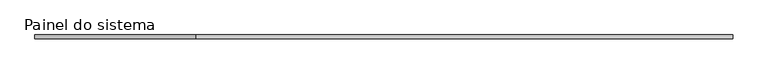
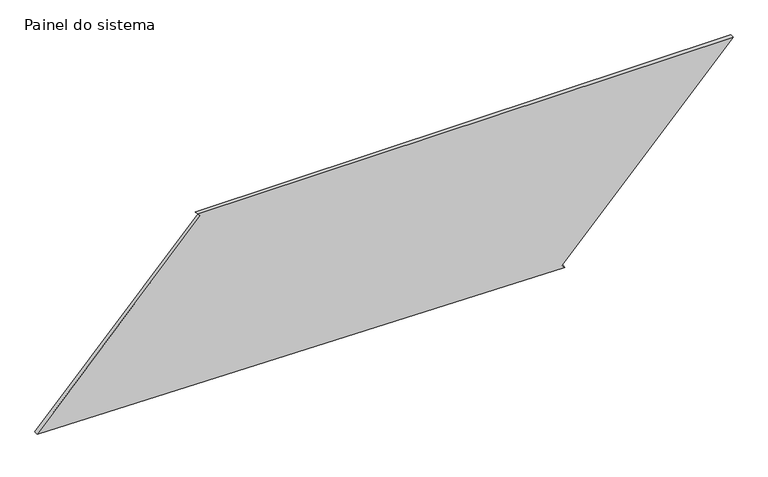
"""IFC4 building model written with IfcOpenShell, lengths in millimetres: plate geometry, Painel do sistema : Envidraçado."""

from ifc_helpers import new_model, si_unit, frame, origin, place, context, project, spatial, polyline, outline, extrude, source, transform, mapped, element, save


def painel_do_sistema_33a86282(model_context):
    return source(origin(), model_context, "Body", "SweptSolid", [
        extrude(outline(polyline([(0.0, 1173.2572083), (17.1196584, 1155.0386108), (1206.0478913, 2272.251125), (1206.0478913, -1223.6668923), (1188.9282329, -1205.4482947), (53.6455649, -2272.251125), (0.0, 1173.2572083)])), frame((0.0, 24.5, 0.0), z_axis=(0.0, 1.0, 0.0), x_axis=(0.0, 0.0, 1.0)), (0.0, 0.0, 1.0), 25.0),
    ])


if __name__ == "__main__":
    model = new_model("IFC4")
    model_context = context("Model", 3, world=origin())
    ifc_project = project(units=[si_unit("LENGTHUNIT", "METRE", prefix="MILLI")], contexts=[model_context])
    site = spatial("IfcSite", under=ifc_project)
    building = spatial("IfcBuilding", under=site)
    placement = place(None, origin())
    painel_do_sistema_shape = painel_do_sistema_33a86282(model_context)
    element("IfcPlate", 1, ObjectType="Painel do sistema : Envidraçado", at=placement, inside=building, context=model_context, shape_type="MappedRepresentation", body=[
        mapped(painel_do_sistema_shape, transform((0.0, 0.0, 0.0), x_axis=(1.0, 0.0, 0.0), y_axis=(0.0, 1.0, 0.0), z_axis=(0.0, 0.0, 1.0))),
    ])
    save(model, "model.ifc")

# Revit data of these elements
# Type "Painel do sistema : Envidraçado"
#   Construction Type Id = "GSP4R"
#   Analytic Construction = "Vidraça única Pilkington 1/8 pol"
#   Visual Light Transmittance = 0.9
#   Solar Heat Gain Coefficient = 0.86
#   Heat Transfer Coefficient (U) = 6.7069 W/(m²·K)
# Element 1 (IfcPlate, "Painel do sistema : Envidraçado")
#   Materials on its faces: "Vidro"
# Materials
#   "Vidro": class "Vidro", colour RGB 0 128 192, transparency 0.9, Description = "Vidro de sílica", Cost = 0
